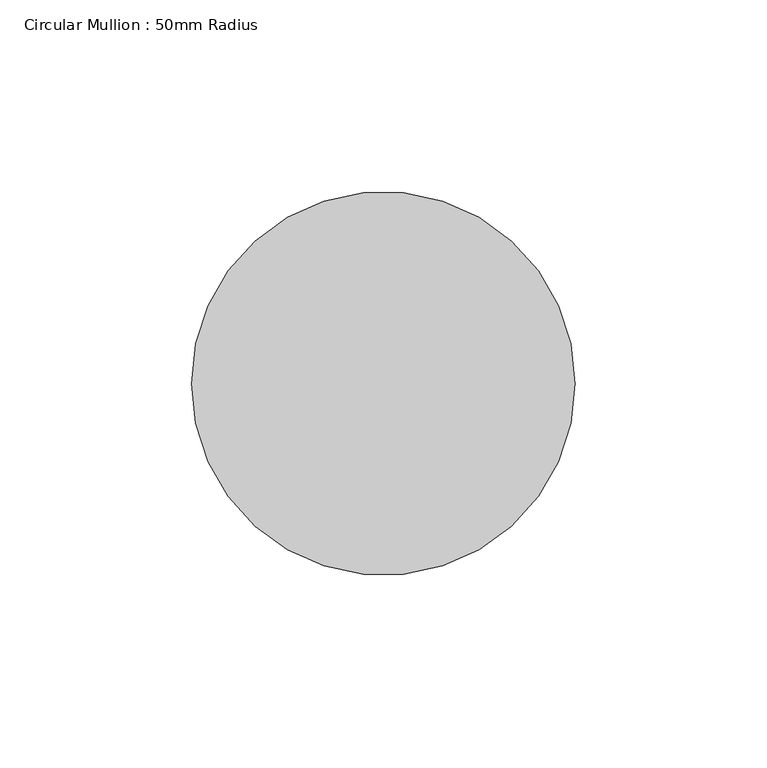
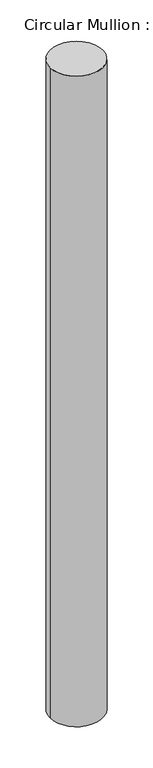
"""IFC4 building model written with IfcOpenShell, lengths in millimetres: member geometry, Circular Mullion : 50mm Radius."""

from ifc_helpers import new_model, si_unit, point, frame, origin, origin_2d, place, context, project, spatial, circle_curve, trimmed, segment, composite_curve, outline, extrude, source, transform, mapped, element, save


def circular_mullion_50mm_radius_736f8f20(model_context):
    return source(origin(), model_context, "Body", "SweptSolid", [
        extrude(outline(composite_curve([segment(trimmed(circle_curve(origin_2d(), 50.0), [point((50.0, 0.0))], [point((-50.0, 0.0))], False, "CARTESIAN"), True, "CONTINUOUS"), segment(trimmed(circle_curve(origin_2d(), 50.0), [point((-50.0, 0.0))], [point((50.0, 0.0))], False, "CARTESIAN"), True, "CONTINUOUS")], self_intersect=False)), frame((0.0, 0.0, -1300.3719501), z_axis=(0.0, 0.0, 1.0), x_axis=(1.0, 0.0, 0.0)), (0.0, 0.0, 1.0), 1300.3719501),
    ])


if __name__ == "__main__":
    model = new_model("IFC4")
    model_context = context("Model", 3, world=origin())
    ifc_project = project(units=[si_unit("LENGTHUNIT", "METRE", prefix="MILLI")], contexts=[model_context])
    site = spatial("IfcSite", under=ifc_project)
    building = spatial("IfcBuilding", under=site)
    placement = place(None, origin())
    circular_mullion_50mm_radius_shape = circular_mullion_50mm_radius_736f8f20(model_context)
    element("IfcMember", 1, ObjectType="Circular Mullion : 50mm Radius", at=placement, inside=building, context=model_context, shape_type="MappedRepresentation", body=[
        mapped(circular_mullion_50mm_radius_shape, transform((0.0, 0.0, 0.0), x_axis=(1.0, 0.0, 0.0), y_axis=(0.0, 1.0, 0.0), z_axis=(0.0, 0.0, 1.0))),
    ])
    save(model, "model.ifc")

# Revit data of these elements
# Type "Circular Mullion : 50mm Radius"
#   built-in parameter 1007350 = 0.164042 (stored number, unit not read)
# Element 1 (IfcMember, "Circular Mullion : 50mm Radius")
#   Materials on its faces: "Aluminium"
# Materials
#   "Aluminium": class "Metal", colour RGB 247 247 247, transparency 0, Description = "Aluminium 6061", Cost = 0
